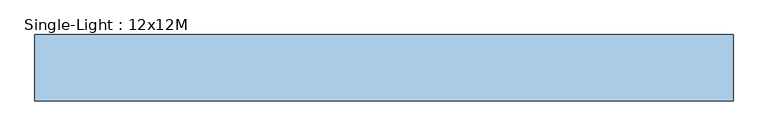
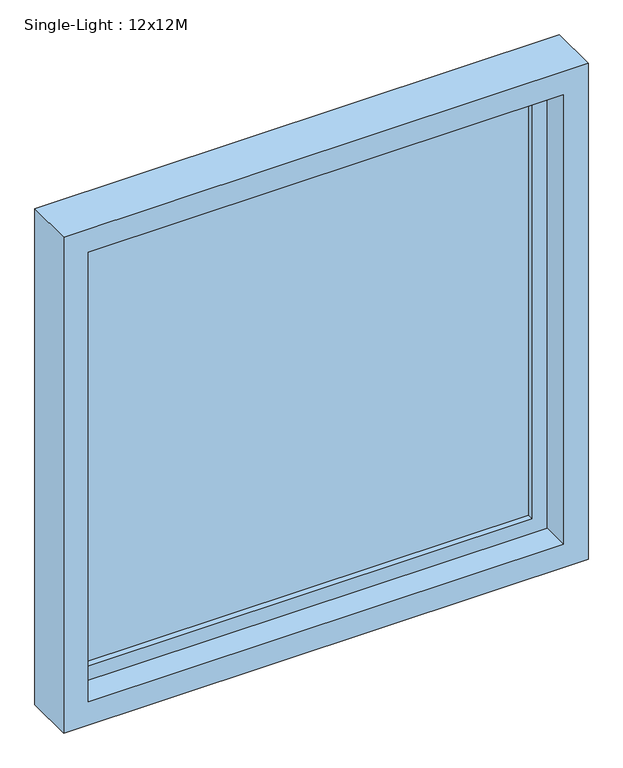
"""IFC4 building model written with IfcOpenShell, lengths in millimetres: window geometry, Single-Light : 12x12M."""

import ifcopenshell
import ifcopenshell.guid

model = None  # the IFC model being written
_history = None  # IfcOwnerHistory: only IFC2X3 demands one
_inside = {}  # id of a spatial element -> (the spatial element, [elements in it])
_under = {}  # id of a project, library or spatial element -> (it, [spatial elements below it])
_declared = {}  # id of a project -> (the project, [libraries it declares])
_typed = {}  # id of a type object -> (the type object, [elements of that type])
_made_of = {}  # id of a material, layer set ... -> (it, [elements and type objects made of it])


def new_model(schema):
    """Start an empty IFC model of exactly this schema.

    Asked for "IFC4X3", IfcOpenShell would pick the latest addendum, in which some entities
    have other attributes; the version numbers below select the first issue.
    IFC2X3 requires an IfcOwnerHistory on every rooted entity: one is made here for all.
    """
    global model, _history
    if schema == "IFC4X3":
        model = ifcopenshell.file(schema_version=(4, 3, 0, 0))
    else:
        model = ifcopenshell.file(schema=schema)
    _inside.clear()
    _under.clear()
    _declared.clear()
    _typed.clear()
    _made_of.clear()
    _history = None
    if model.schema == "IFC2X3":
        org = make("IfcOrganization", Name="unknown")
        user = make(
            "IfcPersonAndOrganization",
            ThePerson=make("IfcPerson", FamilyName="unknown"),
            TheOrganization=org,
        )
        app = make(
            "IfcApplication",
            ApplicationDeveloper=org,
            Version="unknown",
            ApplicationFullName="unknown",
            ApplicationIdentifier="unknown",
        )
        _history = make(
            "IfcOwnerHistory",
            OwningUser=user,
            OwningApplication=app,
            ChangeAction="ADDED",
            CreationDate=0,
        )
    return model


def make(cls, **values):
    """One entity of the class cls with the attributes given. An attribute that is None is left unset."""
    return model.create_entity(
        cls, **{name: value for name, value in values.items() if value is not None}
    )


def rooted(cls, **values):
    """An entity with a GlobalId (a new one), such as an element, a storey or a relation."""
    return make(cls, GlobalId=ifcopenshell.guid.new(), OwnerHistory=_history, **values)


def si_unit(unit_type, name, prefix=None):
    """IfcSIUnit, for example si_unit("LENGTHUNIT", "METRE", prefix="MILLI")."""
    return make("IfcSIUnit", UnitType=unit_type, Prefix=prefix, Name=name)


def assignment(units):
    """IfcUnitAssignment: the units of a project."""
    return None if units is None else make("IfcUnitAssignment", Units=units)


def point(xyz):
    """IfcCartesianPoint."""
    return None if xyz is None else make("IfcCartesianPoint", Coordinates=xyz)


def direction(xyz):
    """IfcDirection."""
    return None if xyz is None else make("IfcDirection", DirectionRatios=xyz)


def frame(location, z_axis=None, x_axis=None):
    """IfcAxis2Placement3D, a coordinate frame: its origin and axes. An axis left out is left unset."""
    return make(
        "IfcAxis2Placement3D",
        Location=point(location),
        Axis=direction(z_axis),
        RefDirection=direction(x_axis),
    )


def origin():
    """The frame at (0, 0, 0) with its axes left unset."""
    return frame((0.0, 0.0, 0.0))


def place(relative_to, where):
    """IfcLocalPlacement: puts the frame where relative to a parent placement (None: the world)."""
    return make(
        "IfcLocalPlacement", PlacementRelTo=relative_to, RelativePlacement=where
    )


def context(
    kind, dimensions, precision=None, world=None, true_north=None, identifier=None
):
    """IfcGeometricRepresentationContext, for example the 3D "Model" context."""
    return make(
        "IfcGeometricRepresentationContext",
        ContextIdentifier=identifier,
        ContextType=kind,
        CoordinateSpaceDimension=dimensions,
        Precision=precision,
        WorldCoordinateSystem=world,
        TrueNorth=true_north,
    )


def project(units=None, contexts=None):
    """IfcProject with its units and contexts."""
    return rooted(
        "IfcProject",
        Name="project",
        RepresentationContexts=contexts,
        UnitsInContext=assignment(units),
    )


def spatial(cls, under=None, at=None, **own):
    """A site, building, storey or space (cls), placed at a placement, below another one or the project."""
    s = rooted(cls, ObjectPlacement=at, **own)
    if under is not None:
        _under.setdefault(under.id(), (under, []))[1].append(s)
    return s


def polyline(points):
    """IfcPolyline through the points."""
    return make("IfcPolyline", Points=[point(p) for p in points])


def outline(outer, holes=None, kind="AREA"):
    """IfcArbitraryClosedProfileDef: a profile drawn as a closed curve; with holes, ...WithVoids."""
    if holes is None:
        return make("IfcArbitraryClosedProfileDef", ProfileType=kind, OuterCurve=outer)
    return make(
        "IfcArbitraryProfileDefWithVoids",
        ProfileType=kind,
        OuterCurve=outer,
        InnerCurves=holes,
    )


def extrude(swept, where, along, depth):
    """IfcExtrudedAreaSolid: the profile swept, set in the frame where, extruded along a direction by depth."""
    return make(
        "IfcExtrudedAreaSolid",
        SweptArea=swept,
        Position=where,
        ExtrudedDirection=direction(along),
        Depth=depth,
    )


def faces_of(points, faces, orient=None, outer=None):
    """IfcFace entities. A face is a list of loops; a loop is a list of indices into points, from 0.

    orient and outer hold one flag for each loop. By default every Orientation is true, the
    first loop of a face is its IfcFaceOuterBound and the others are IfcFaceBound.
    """
    made = []
    for i, loops in enumerate(faces):
        bounds = []
        for j, loop in enumerate(loops):
            is_outer = j == 0 if outer is None else outer[i][j]
            bounds.append(
                make(
                    "IfcFaceOuterBound" if is_outer else "IfcFaceBound",
                    Bound=make("IfcPolyLoop", Polygon=[points[k] for k in loop]),
                    Orientation=True if orient is None else orient[i][j],
                )
            )
        made.append(make("IfcFace", Bounds=bounds))
    return made


def faceted_brep(points, faces, orient=None, outer=None, voids=None):
    """IfcFacetedBrep: a solid bounded by flat faces; with voids (closed shells), ...WithVoids."""
    shared = [point(p) for p in points]
    hull = make("IfcClosedShell", CfsFaces=faces_of(shared, faces, orient, outer))
    if voids is None:
        return make("IfcFacetedBrep", Outer=hull)
    return make(
        "IfcFacetedBrepWithVoids",
        Outer=hull,
        Voids=[
            make(cls, CfsFaces=faces_of(shared, fs, o, b)) for cls, fs, o, b in voids
        ],
    )


def shape(context_of_items, identifier, shape_type, items):
    """IfcShapeRepresentation: the items that make up one representation, for example the "Body"."""
    return make(
        "IfcShapeRepresentation",
        ContextOfItems=context_of_items,
        RepresentationIdentifier=identifier,
        RepresentationType=shape_type,
        Items=items,
    )


def source(mapping_origin, context_of_items, identifier, shape_type, items):
    """IfcRepresentationMap: a shape defined once, which mapped items show again and again."""
    return make(
        "IfcRepresentationMap",
        MappingOrigin=mapping_origin,
        MappedRepresentation=shape(context_of_items, identifier, shape_type, items),
    )


def transform(
    local_origin,
    x_axis=None,
    y_axis=None,
    z_axis=None,
    scale=None,
    scale2=None,
    scale3=None,
    uniform=True,
):
    """IfcCartesianTransformationOperator3D, or its non-uniform kind. x_axis, y_axis, z_axis: its Axis1, 2, 3."""
    if uniform:
        return make(
            "IfcCartesianTransformationOperator3D",
            Axis1=direction(x_axis),
            Axis2=direction(y_axis),
            LocalOrigin=point(local_origin),
            Scale=scale,
            Axis3=direction(z_axis),
        )
    return make(
        "IfcCartesianTransformationOperator3DnonUniform",
        Axis1=direction(x_axis),
        Axis2=direction(y_axis),
        LocalOrigin=point(local_origin),
        Scale=scale,
        Axis3=direction(z_axis),
        Scale2=scale2,
        Scale3=scale3,
    )


def mapped(mapping_source, mapping_target):
    """IfcMappedItem: shows the shape of a source again, moved by a transform."""
    return make(
        "IfcMappedItem", MappingSource=mapping_source, MappingTarget=mapping_target
    )


def made_of(thing, what):
    """Note that an element or type object is made of a material, layer set ...; save() writes the relation."""
    if what is not None:
        _made_of.setdefault(what.id(), (what, []))[1].append(thing)
    return thing


def element(
    cls,
    number,
    at=None,
    inside=None,
    cuts=None,
    type_object=None,
    material=None,
    context=None,
    identifier="Body",
    shape_type=None,
    held_by="IfcProductDefinitionShape",
    body=None,
    shapes=None,
    **own,
):
    """One element of the class cls, such as IfcWall. Its Tag is "e" and its number.

    at: its placement. inside: the storey or other place that contains it. cuts: it is an
    opening in that element (IfcRelVoidsElement). A single representation is given by context,
    identifier, shape_type and body (its items); several are given by shapes. held_by: the class
    of the entity that holds the representations. save() writes the other relations.
    """
    e = rooted(cls, Tag="e%d" % number, ObjectPlacement=at, **own)
    if body is not None:
        shapes = [shape(context, identifier, shape_type, body)]
    if shapes is not None:
        e.Representation = make(held_by, Representations=shapes)
    if inside is not None:
        _inside.setdefault(inside.id(), (inside, []))[1].append(e)
    if cuts is not None:
        rooted(
            "IfcRelVoidsElement", RelatingBuildingElement=cuts, RelatedOpeningElement=e
        )
    if type_object is not None:
        _typed.setdefault(type_object.id(), (type_object, []))[1].append(e)
    return made_of(e, material)


def aggregate(whole, parts):
    """IfcRelAggregates: a whole, such as a stair, and the parts it consists of."""
    return rooted("IfcRelAggregates", RelatingObject=whole, RelatedObjects=parts)


def save(model, path):
    """Write the relations noted so far, then the file.

    IfcRelAggregates (storeys below a building ...), IfcRelContainedInSpatialStructure (elements
    in a storey), IfcRelDefinesByType, IfcRelAssociatesMaterial and IfcRelDeclares: one each for
    every whole, place, type object, material and project.
    """
    for whole, parts in _under.values():
        aggregate(whole, parts)
    for where, things in _inside.values():
        rooted(
            "IfcRelContainedInSpatialStructure",
            RelatedElements=things,
            RelatingStructure=where,
        )
    for kind, things in _typed.values():
        rooted("IfcRelDefinesByType", RelatedObjects=things, RelatingType=kind)
    for what, things in _made_of.values():
        rooted("IfcRelAssociatesMaterial", RelatedObjects=things, RelatingMaterial=what)
    for by, libraries in _declared.values():
        rooted("IfcRelDeclares", RelatingContext=by, RelatedDefinitions=libraries)
    model.write(path)


def single_light_12x12m_8659da90(model_context):
    return source(origin(), model_context, "Body", "SolidModel", [
        extrude(outline(polyline([(1970.0, -564.0), (842.0, -564.0), (842.0, 564.0), (1970.0, 564.0), (1970.0, -564.0)]), holes=[polyline([(1920.0, 514.0), (892.0, 514.0), (892.0, -514.0), (1920.0, -514.0), (1920.0, 514.0)])]), frame((0.0, 134.0, 0.0), z_axis=(0.0, 1.0, 0.0), x_axis=(0.0, 0.0, 1.0)), (0.0, 0.0, 1.0), 50.0),
        faceted_brep([(-606.0, 69.0, 800.0), (-606.0, 184.0, 800.0), (606.0, 184.0, 800.0), (606.0, 69.0, 800.0), (606.0, 184.0, 2012.0), (606.0, 69.0, 2012.0), (-606.0, 184.0, 2012.0), (564.0, 184.0, 1970.0), (-564.0, 184.0, 1970.0), (-564.0, 184.0, 842.0), (564.0, 184.0, 842.0), (-606.0, 69.0, 2012.0), (549.0, 69.0, 857.0), (-549.0, 69.0, 857.0), (-549.0, 69.0, 1955.0), (549.0, 69.0, 1955.0), (-549.0, 134.0, 857.0), (549.0, 134.0, 857.0), (549.0, 134.0, 1955.0), (564.0, 134.0, 842.0), (-564.0, 134.0, 842.0), (-564.0, 134.0, 1970.0), (564.0, 134.0, 1970.0), (-549.0, 134.0, 1955.0)], [[[0, 1, 2, 3]], [[3, 2, 4, 5]], [[2, 1, 6, 4], [7, 8, 9, 10]], [[5, 11, 0, 3], [12, 13, 14, 15]], [[16, 13, 12, 17]], [[17, 12, 15, 18]], [[19, 20, 21, 22], [18, 23, 16, 17]], [[9, 20, 19, 10]], [[10, 19, 22, 7]], [[11, 6, 1, 0]], [[23, 14, 13, 16]], [[8, 21, 20, 9]], [[5, 4, 6, 11]], [[18, 15, 14, 23]], [[7, 22, 21, 8]]]),
        extrude(outline(polyline([(-514.0, 170.0), (514.0, 170.0), (514.0, 148.0), (-514.0, 148.0), (-514.0, 170.0)])), frame((0.0, 0.0, 892.0), z_axis=(0.0, 0.0, 1.0), x_axis=(1.0, 0.0, 0.0)), (0.0, 0.0, 1.0), 1028.0),
    ])


if __name__ == "__main__":
    model = new_model("IFC4")
    model_context = context("Model", 3, world=origin())
    ifc_project = project(units=[si_unit("LENGTHUNIT", "METRE", prefix="MILLI")], contexts=[model_context])
    site = spatial("IfcSite", under=ifc_project)
    building = spatial("IfcBuilding", under=site)
    placement = place(None, origin())
    single_light_12x12m_shape = single_light_12x12m_8659da90(model_context)
    element("IfcWindow", 1, ObjectType="Single-Light : 12x12M", at=placement, inside=building, context=model_context, shape_type="MappedRepresentation", body=[
        mapped(single_light_12x12m_shape, transform((0.0, 0.0, 0.0), x_axis=(1.0, 0.0, 0.0), y_axis=(0.0, 1.0, 0.0), z_axis=(0.0, 0.0, 1.0))),
    ])
    save(model, "model.ifc")

# Revit data of these elements
# Type "Single-Light : 12x12M"
#   Type Mark = "39"
#   Creator Organization [instance default] = "© Danish Educational Content"
#   Creator Name [instance default] = "© Erik Falck Jørgensen"
#   Creator Build [instance default] = "2017.0801.0"
#   Analytic Construction = "<None>"
#   length#5 = -36 mm
#   length#4 = -14 mm
#   length#3 = 120 mm
#   length#2 = 57 mm
#   length#1 = 0 mm
#   Seal Width = 12 mm
#   Rough Width = 1212 mm
#   Rough Height = 1212 mm
#   Rebate Depth = 50 mm
#   Rabbet Width = 15 mm
#   Rabbet Depth = 50 mm
#   Height = 1188 mm
#   Glass Thickness = 22 mm
#   Frame Width = 50 mm
#   Frame Depth = 50 mm
#   Exterior Direction [instance default] = 0.00°
#   Case Depth = 115 mm
#   Case Width = 45 mm
#   Default Sill Height = 800 mm
#   Width = 1188 mm
#   Sealing = no
#   Hinging = yes
#   Wall Closure = 1
#   Above Cutplane [instance default] = no
#   Wall Surface = none
#   Sill Plate = none
#   Glass = none
#   Frame/Mullion = none
#   Embrasure = none
#   Case/Transom = none
# Element 1 (IfcWindow, "Single-Light : 12x12M")
#   Materials on its faces: "Default Frame/Mullion (Interior/Exterior)", "Glass"
# Materials
#   "Default Frame/Mullion (Interior/Exterior)": class "Generic", colour RGB 205 205 205, transparency 0, Description = "Udefineret karm/ramme materiale", Cost = 0
#   "Glass": class "Glass", colour RGB 180 200 255, transparency 0.75, Description = "Generisk glas", Cost = 0
